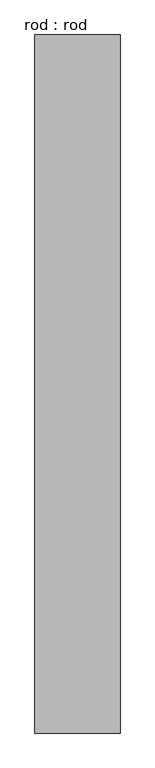
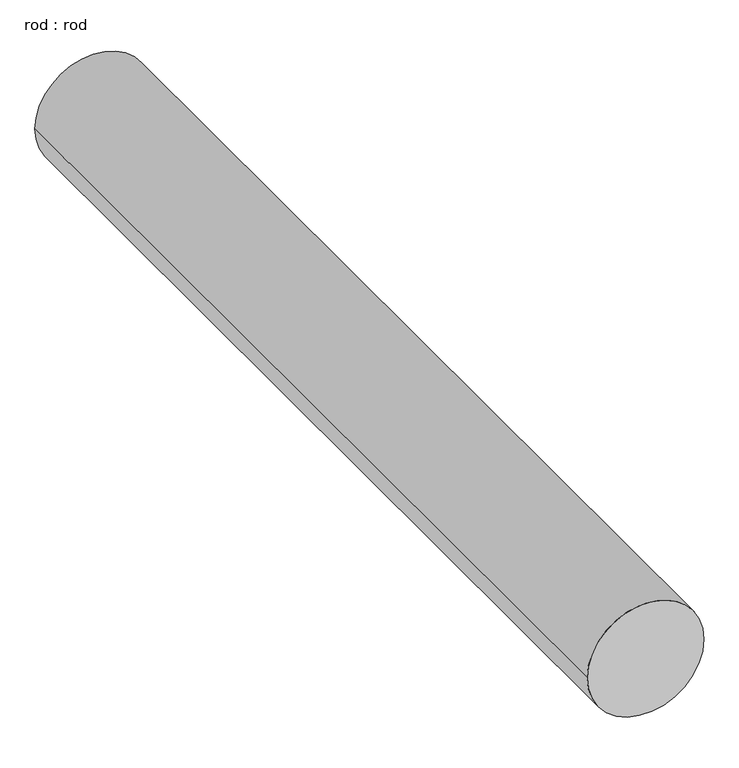
"""IFC4 building model written with IfcOpenShell, lengths in millimetres: proxy geometry, rod : rod."""

from ifc_helpers import new_model, si_unit, point, frame, frame_2d, origin, place, context, project, spatial, circle_curve, trimmed, segment, composite_curve, outline, extrude, source, transform, mapped, element, save


def rod_rod_567c912b(model_context):
    return source(origin(), model_context, "Body", "SweptSolid", [
        extrude(outline(composite_curve([segment(trimmed(circle_curve(frame_2d((0.0108462, 0.0)), 200.0), [point((0.0108462, 200.0))], [point((0.0108462, -200.0))], False, "CARTESIAN"), True, "CONTINUOUS"), segment(trimmed(circle_curve(frame_2d((0.0108462, 0.0)), 200.0), [point((0.0108462, -200.0))], [point((0.0108462, 200.0))], False, "CARTESIAN"), True, "CONTINUOUS")], self_intersect=False)), frame((0.0, 2453.4429011, 0.0), z_axis=(0.0, 1.0, 0.0), x_axis=(0.0, 0.0, 1.0)), (0.0, 0.0, 1.0), 3278.5714286),
    ])


if __name__ == "__main__":
    model = new_model("IFC4")
    model_context = context("Model", 3, world=origin())
    ifc_project = project(units=[si_unit("LENGTHUNIT", "METRE", prefix="MILLI")], contexts=[model_context])
    site = spatial("IfcSite", under=ifc_project)
    building = spatial("IfcBuilding", under=site)
    placement = place(None, origin())
    rod_rod_shape = rod_rod_567c912b(model_context)
    element("IfcBuildingElementProxy", 1, Name="rod : rod", ObjectType="rod : rod", at=placement, inside=building, context=model_context, shape_type="MappedRepresentation", body=[
        mapped(rod_rod_shape, transform((0.0, 0.0, 0.0), x_axis=(1.0, 0.0, 0.0), y_axis=(0.0, 1.0, 0.0), z_axis=(0.0, 0.0, 1.0))),
    ])
    save(model, "model.ifc")

# Revit data of these elements
# Type "rod : rod"
#   Default Elevation = 0
